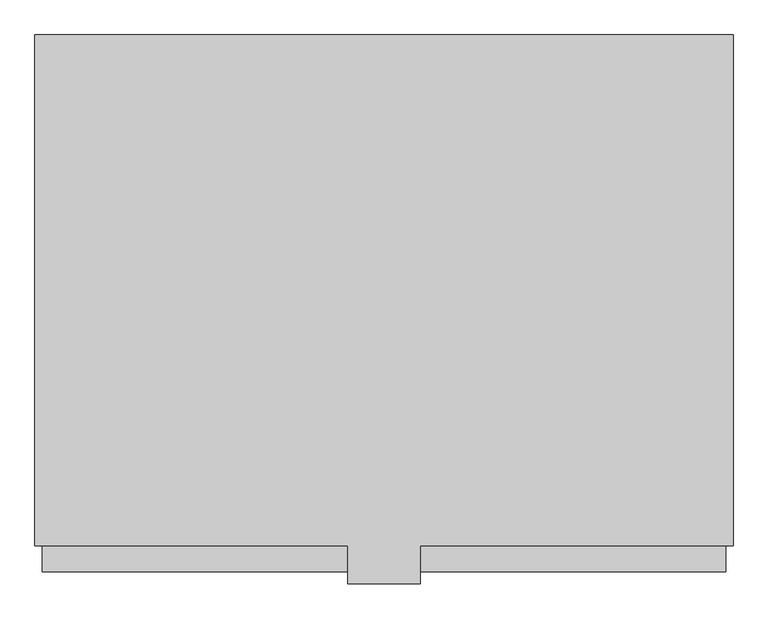
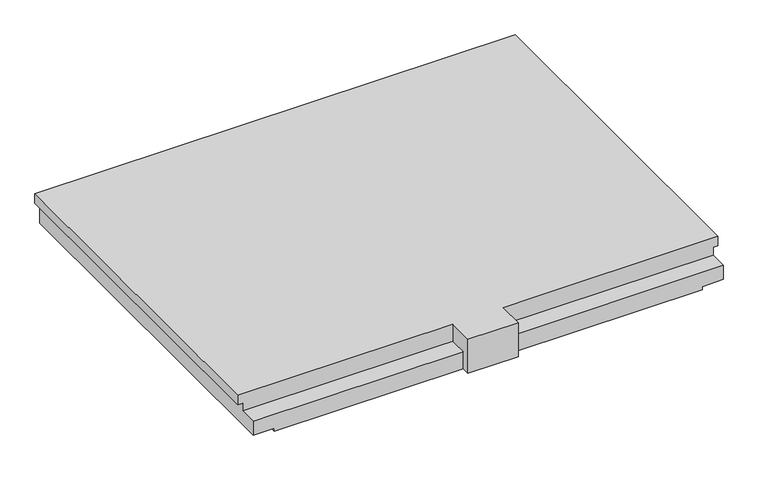
"""IFC4 building model written with IfcOpenShell, lengths in millimetres: stair geometry, NLRS_24_GM_UN_rechthoekig bordes prefab-AV_gen_rsf : prefab bordes_gen__2250x2925."""

from ifc_helpers import new_model, si_unit, origin, place, context, project, spatial, faceted_brep, source, transform, mapped, element, save


def stair_ecb21330(model_context):
    return source(origin(), model_context, "Body", "Brep", [
        faceted_brep([(1462.5, -2140.0, 0.0), (1462.5, -2140.0, -60.0), (1462.5, 0.0, -60.0), (1462.5, 0.0, 0.0), (152.5, -2250.0, -110.0), (1432.5, -2250.0, -110.0), (1432.5, -2140.0, -110.0), (152.5, -2140.0, -110.0), (152.5, -2140.0, 0.0), (1432.5, -2140.0, -60.0), (152.5, -2300.0, -220.0), (152.5, -2250.0, -220.0), (152.5, -2300.0, 0.0), (-152.5, -2300.0, 0.0), (-152.5, -2140.0, 0.0), (-152.5, -2140.0, -110.0), (-152.5, -2250.0, -110.0), (-152.5, -2250.0, -220.0), (-152.5, -2300.0, -220.0), (-1462.5, 0.0, 0.0), (-1462.5, 0.0, -60.0), (-1462.5, -2140.0, -60.0), (-1462.5, -2140.0, 0.0), (-1432.5, -2250.0, -110.0), (-1432.5, -2250.0, -200.0), (-1302.5, -2250.0, -200.0), (-1302.5, -2250.0, -220.0), (-1432.5, -2140.0, -110.0), (-1432.5, -2140.0, -60.0), (1432.5, 0.0, -60.0), (1432.5, 0.0, -200.0), (1302.5, 0.0, -200.0), (1302.5, 0.0, -220.0), (-1302.5, 0.0, -220.0), (-1302.5, 0.0, -200.0), (-1432.5, 0.0, -200.0), (-1432.5, 0.0, -60.0), (1302.5, -2250.0, -220.0), (1432.5, -2250.0, -200.0), (1302.5, -2250.0, -200.0)], [[[0, 1, 2, 3]], [[4, 5, 6, 7]], [[8, 7, 6, 9, 1, 0]], [[10, 11, 4, 7, 8, 12]], [[13, 14, 15, 16, 17, 18]], [[19, 20, 21, 22]], [[17, 16, 23, 24, 25, 26]], [[16, 15, 27, 23]], [[22, 21, 28, 27, 15, 14]], [[22, 14, 13, 12, 8, 0, 3, 19]], [[19, 3, 2, 29, 30, 31, 32, 33, 34, 35, 36, 20]], [[26, 33, 32, 37, 11, 10, 18, 17]], [[28, 21, 20, 36]], [[24, 23, 27, 28, 36, 35]], [[35, 34, 25, 24]], [[34, 33, 26, 25]], [[29, 2, 1, 9]], [[9, 6, 5, 38, 30, 29]], [[38, 39, 31, 30]], [[39, 37, 32, 31]], [[11, 37, 39, 38, 5, 4]], [[12, 13, 18, 10]]]),
    ])


if __name__ == "__main__":
    model = new_model("IFC4")
    model_context = context("Model", 3, world=origin())
    ifc_project = project(units=[si_unit("LENGTHUNIT", "METRE", prefix="MILLI")], contexts=[model_context])
    site = spatial("IfcSite", under=ifc_project)
    building = spatial("IfcBuilding", under=site)
    placement = place(None, origin())
    stair_shape = stair_ecb21330(model_context)
    element("IfcStair", 1, ObjectType="NLRS_24_GM_UN_rechthoekig bordes prefab-AV_gen_rsf : prefab bordes_gen__2250x2925", at=placement, inside=building, context=model_context, shape_type="MappedRepresentation", body=[
        mapped(stair_shape, transform((0.0, 0.0, 0.0), x_axis=(1.0, 0.0, 0.0), y_axis=(0.0, 1.0, 0.0), z_axis=(0.0, 0.0, 1.0))),
    ])
    save(model, "model.ifc")

# Revit data of these elements
# Type "NLRS_24_GM_UN_rechthoekig bordes prefab-AV_gen_rsf : prefab bordes_gen__2250x2925"
#   IfcExportAs = "IfcStair"
#   Type Comments = " "
#   Model = " "
#   Manufacturer = " "
#   Description = "rechthoekig bordes prefab\r\n1930x4395"
#   Assembly Code = "24.15"
#   Width = 2925 mm
#   Thickness = 220 mm
#   Perimeter = 10450 mm
#   NLRS_C_lengte_02 = 1310 mm
#   NLRS_C_lengte_01 = 1310 mm
#   NLRS_C_hoogte_02 = 110 mm
#   NLRS_C_hoogte_01 = 110 mm
#   NLRS_C_diepte_04 = 2250 mm
#   NLRS_C_diepte_03 = 2250 mm
#   NLRS_C_diepte_02 = 110 mm
#   NLRS_C_diepte_01 = 110 mm
#   Length = 2300 mm
#   Default Elevation = 1219.2 mm
#   Area = 6.7275 m²
#   NLRS_C_materiaal = NLRS_f2_beton prefab_gen_rsf
#   Keynote = ""
# Element 1 (IfcStair, "NLRS_24_GM_UN_rechthoekig bordes prefab-AV_gen_rsf : prefab bordes_gen__2250x2925")
#   Materials on its faces: "NLRS_f2_beton prefab_gen_rsf"
# Materials
#   "NLRS_f2_beton prefab_gen_rsf": class "F - Niet gebakken kunststeen", colour RGB 129 133 118, transparency 0, Keynote = "f2", Manufacturer = "Revit Standards Foundation", URL = "www.revitstandards.org", Description = "beton prefab", Cost = 0
